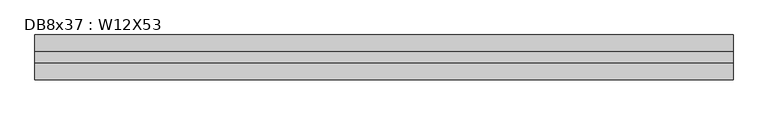
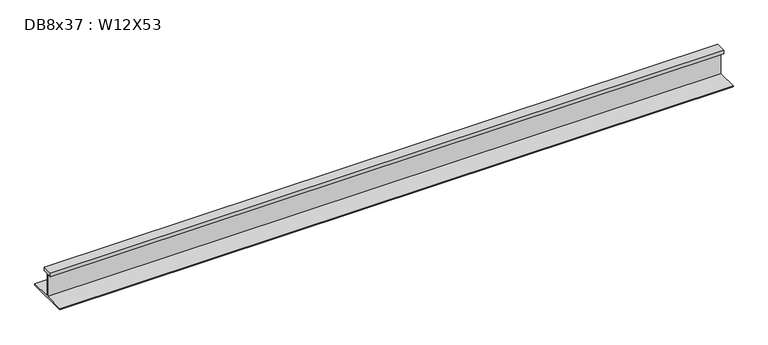
"""IFC4 building model written with IfcOpenShell, lengths in millimetres: beam geometry, DB8x37 : W12X53."""

import ifcopenshell
import ifcopenshell.guid

model = None  # the IFC model being written
_history = None  # IfcOwnerHistory: only IFC2X3 demands one
_inside = {}  # id of a spatial element -> (the spatial element, [elements in it])
_under = {}  # id of a project, library or spatial element -> (it, [spatial elements below it])
_declared = {}  # id of a project -> (the project, [libraries it declares])
_typed = {}  # id of a type object -> (the type object, [elements of that type])
_made_of = {}  # id of a material, layer set ... -> (it, [elements and type objects made of it])


def new_model(schema):
    """Start an empty IFC model of exactly this schema.

    Asked for "IFC4X3", IfcOpenShell would pick the latest addendum, in which some entities
    have other attributes; the version numbers below select the first issue.
    IFC2X3 requires an IfcOwnerHistory on every rooted entity: one is made here for all.
    """
    global model, _history
    if schema == "IFC4X3":
        model = ifcopenshell.file(schema_version=(4, 3, 0, 0))
    else:
        model = ifcopenshell.file(schema=schema)
    _inside.clear()
    _under.clear()
    _declared.clear()
    _typed.clear()
    _made_of.clear()
    _history = None
    if model.schema == "IFC2X3":
        org = make("IfcOrganization", Name="unknown")
        user = make(
            "IfcPersonAndOrganization",
            ThePerson=make("IfcPerson", FamilyName="unknown"),
            TheOrganization=org,
        )
        app = make(
            "IfcApplication",
            ApplicationDeveloper=org,
            Version="unknown",
            ApplicationFullName="unknown",
            ApplicationIdentifier="unknown",
        )
        _history = make(
            "IfcOwnerHistory",
            OwningUser=user,
            OwningApplication=app,
            ChangeAction="ADDED",
            CreationDate=0,
        )
    return model


def make(cls, **values):
    """One entity of the class cls with the attributes given. An attribute that is None is left unset."""
    return model.create_entity(
        cls, **{name: value for name, value in values.items() if value is not None}
    )


def rooted(cls, **values):
    """An entity with a GlobalId (a new one), such as an element, a storey or a relation."""
    return make(cls, GlobalId=ifcopenshell.guid.new(), OwnerHistory=_history, **values)


def si_unit(unit_type, name, prefix=None):
    """IfcSIUnit, for example si_unit("LENGTHUNIT", "METRE", prefix="MILLI")."""
    return make("IfcSIUnit", UnitType=unit_type, Prefix=prefix, Name=name)


def assignment(units):
    """IfcUnitAssignment: the units of a project."""
    return None if units is None else make("IfcUnitAssignment", Units=units)


def point(xyz):
    """IfcCartesianPoint."""
    return None if xyz is None else make("IfcCartesianPoint", Coordinates=xyz)


def direction(xyz):
    """IfcDirection."""
    return None if xyz is None else make("IfcDirection", DirectionRatios=xyz)


def frame(location, z_axis=None, x_axis=None):
    """IfcAxis2Placement3D, a coordinate frame: its origin and axes. An axis left out is left unset."""
    return make(
        "IfcAxis2Placement3D",
        Location=point(location),
        Axis=direction(z_axis),
        RefDirection=direction(x_axis),
    )


def origin():
    """The frame at (0, 0, 0) with its axes left unset."""
    return frame((0.0, 0.0, 0.0))


def place(relative_to, where):
    """IfcLocalPlacement: puts the frame where relative to a parent placement (None: the world)."""
    return make(
        "IfcLocalPlacement", PlacementRelTo=relative_to, RelativePlacement=where
    )


def context(
    kind, dimensions, precision=None, world=None, true_north=None, identifier=None
):
    """IfcGeometricRepresentationContext, for example the 3D "Model" context."""
    return make(
        "IfcGeometricRepresentationContext",
        ContextIdentifier=identifier,
        ContextType=kind,
        CoordinateSpaceDimension=dimensions,
        Precision=precision,
        WorldCoordinateSystem=world,
        TrueNorth=true_north,
    )


def project(units=None, contexts=None):
    """IfcProject with its units and contexts."""
    return rooted(
        "IfcProject",
        Name="project",
        RepresentationContexts=contexts,
        UnitsInContext=assignment(units),
    )


def spatial(cls, under=None, at=None, **own):
    """A site, building, storey or space (cls), placed at a placement, below another one or the project."""
    s = rooted(cls, ObjectPlacement=at, **own)
    if under is not None:
        _under.setdefault(under.id(), (under, []))[1].append(s)
    return s


def polyline(points):
    """IfcPolyline through the points."""
    return make("IfcPolyline", Points=[point(p) for p in points])


def outline(outer, holes=None, kind="AREA"):
    """IfcArbitraryClosedProfileDef: a profile drawn as a closed curve; with holes, ...WithVoids."""
    if holes is None:
        return make("IfcArbitraryClosedProfileDef", ProfileType=kind, OuterCurve=outer)
    return make(
        "IfcArbitraryProfileDefWithVoids",
        ProfileType=kind,
        OuterCurve=outer,
        InnerCurves=holes,
    )


def extrude(swept, where, along, depth):
    """IfcExtrudedAreaSolid: the profile swept, set in the frame where, extruded along a direction by depth."""
    return make(
        "IfcExtrudedAreaSolid",
        SweptArea=swept,
        Position=where,
        ExtrudedDirection=direction(along),
        Depth=depth,
    )


def shape(context_of_items, identifier, shape_type, items):
    """IfcShapeRepresentation: the items that make up one representation, for example the "Body"."""
    return make(
        "IfcShapeRepresentation",
        ContextOfItems=context_of_items,
        RepresentationIdentifier=identifier,
        RepresentationType=shape_type,
        Items=items,
    )


def source(mapping_origin, context_of_items, identifier, shape_type, items):
    """IfcRepresentationMap: a shape defined once, which mapped items show again and again."""
    return make(
        "IfcRepresentationMap",
        MappingOrigin=mapping_origin,
        MappedRepresentation=shape(context_of_items, identifier, shape_type, items),
    )


def transform(
    local_origin,
    x_axis=None,
    y_axis=None,
    z_axis=None,
    scale=None,
    scale2=None,
    scale3=None,
    uniform=True,
):
    """IfcCartesianTransformationOperator3D, or its non-uniform kind. x_axis, y_axis, z_axis: its Axis1, 2, 3."""
    if uniform:
        return make(
            "IfcCartesianTransformationOperator3D",
            Axis1=direction(x_axis),
            Axis2=direction(y_axis),
            LocalOrigin=point(local_origin),
            Scale=scale,
            Axis3=direction(z_axis),
        )
    return make(
        "IfcCartesianTransformationOperator3DnonUniform",
        Axis1=direction(x_axis),
        Axis2=direction(y_axis),
        LocalOrigin=point(local_origin),
        Scale=scale,
        Axis3=direction(z_axis),
        Scale2=scale2,
        Scale3=scale3,
    )


def mapped(mapping_source, mapping_target):
    """IfcMappedItem: shows the shape of a source again, moved by a transform."""
    return make(
        "IfcMappedItem", MappingSource=mapping_source, MappingTarget=mapping_target
    )


def made_of(thing, what):
    """Note that an element or type object is made of a material, layer set ...; save() writes the relation."""
    if what is not None:
        _made_of.setdefault(what.id(), (what, []))[1].append(thing)
    return thing


def element(
    cls,
    number,
    at=None,
    inside=None,
    cuts=None,
    type_object=None,
    material=None,
    context=None,
    identifier="Body",
    shape_type=None,
    held_by="IfcProductDefinitionShape",
    body=None,
    shapes=None,
    **own,
):
    """One element of the class cls, such as IfcWall. Its Tag is "e" and its number.

    at: its placement. inside: the storey or other place that contains it. cuts: it is an
    opening in that element (IfcRelVoidsElement). A single representation is given by context,
    identifier, shape_type and body (its items); several are given by shapes. held_by: the class
    of the entity that holds the representations. save() writes the other relations.
    """
    e = rooted(cls, Tag="e%d" % number, ObjectPlacement=at, **own)
    if body is not None:
        shapes = [shape(context, identifier, shape_type, body)]
    if shapes is not None:
        e.Representation = make(held_by, Representations=shapes)
    if inside is not None:
        _inside.setdefault(inside.id(), (inside, []))[1].append(e)
    if cuts is not None:
        rooted(
            "IfcRelVoidsElement", RelatingBuildingElement=cuts, RelatedOpeningElement=e
        )
    if type_object is not None:
        _typed.setdefault(type_object.id(), (type_object, []))[1].append(e)
    return made_of(e, material)


def aggregate(whole, parts):
    """IfcRelAggregates: a whole, such as a stair, and the parts it consists of."""
    return rooted("IfcRelAggregates", RelatingObject=whole, RelatedObjects=parts)


def save(model, path):
    """Write the relations noted so far, then the file.

    IfcRelAggregates (storeys below a building ...), IfcRelContainedInSpatialStructure (elements
    in a storey), IfcRelDefinesByType, IfcRelAssociatesMaterial and IfcRelDeclares: one each for
    every whole, place, type object, material and project.
    """
    for whole, parts in _under.values():
        aggregate(whole, parts)
    for where, things in _inside.values():
        rooted(
            "IfcRelContainedInSpatialStructure",
            RelatedElements=things,
            RelatingStructure=where,
        )
    for kind, things in _typed.values():
        rooted("IfcRelDefinesByType", RelatedObjects=things, RelatingType=kind)
    for what, things in _made_of.values():
        rooted("IfcRelAssociatesMaterial", RelatedObjects=things, RelatingMaterial=what)
    for by, libraries in _declared.values():
        rooted("IfcRelDeclares", RelatingContext=by, RelatedDefinitions=libraries)
    model.write(path)


def db8x37_w12x53_edb2ace5(model_context):
    return source(origin(), model_context, "Body", "SweptSolid", [
        extrude(outline(polyline([(38.1, 145.415), (38.1, 120.015), (2.921, 120.015), (2.921, -48.4505), (152.4, -48.4505), (152.4, -58.1025), (-152.4, -58.1025), (-152.4, -48.4505), (-2.921, -48.4505), (-2.921, 120.015), (-38.1, 120.015), (-38.1, 145.415), (38.1, 145.415)])), frame((-2391.029, 0.0, 0.0), z_axis=(1.0, 0.0, 0.0), x_axis=(0.0, 1.0, 0.0)), (0.0, 0.0, 1.0), 4751.959),
    ])


if __name__ == "__main__":
    model = new_model("IFC4")
    model_context = context("Model", 3, world=origin())
    ifc_project = project(units=[si_unit("LENGTHUNIT", "METRE", prefix="MILLI")], contexts=[model_context])
    site = spatial("IfcSite", under=ifc_project)
    building = spatial("IfcBuilding", under=site)
    placement = place(None, origin())
    db8x37_w12x53_shape = db8x37_w12x53_edb2ace5(model_context)
    element("IfcBeam", 1, ObjectType="DB8x37 : W12X53", at=placement, inside=building, context=model_context, shape_type="MappedRepresentation", body=[
        mapped(db8x37_w12x53_shape, transform((0.0, 0.0, 0.0), x_axis=(1.0, 0.0, 0.0), y_axis=(0.0, 1.0, 0.0), z_axis=(0.0, 0.0, 1.0))),
    ])
    save(model, "model.ifc")

# Revit data of these elements
# Type "DB8x37 : W12X53"
#   Assembly Code = "B10"
#   W = 53
#   Length [instance default] = 5' - 0"
#   bf = 0' - 10"
#   d = 1' - 0.1"
#   k = 0' - 1 3/8"
#   k2 = 0' - 0.8"
#   tf = 0' - 0.575"
#   tw = 0' - 0.345"
#   A = 0.108333 SF
#   Structural Material [instance default] = Steel ASTM A992
# Element 1 (IfcBeam, "DB8x37 : W12X53")
#   Materials on its faces: "Steel ASTM A992"
# Materials
#   "Steel ASTM A992": class "Metal", colour RGB 199 199 199, transparency 0, Description = "Structural steel 50ksi", Cost = 0
